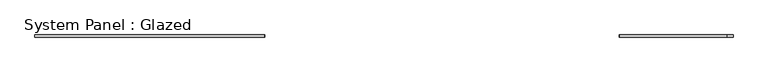
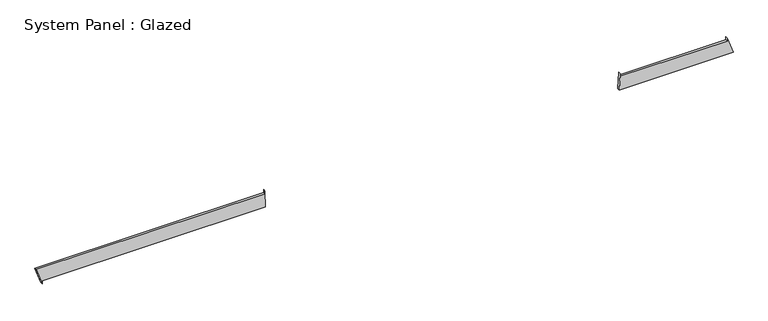
"""IFC4 building model written with IfcOpenShell, lengths in millimetres: plate geometry, System Panel : Glazed."""

import ifcopenshell
import ifcopenshell.guid

model = None  # the IFC model being written
_history = None  # IfcOwnerHistory: only IFC2X3 demands one
_inside = {}  # id of a spatial element -> (the spatial element, [elements in it])
_under = {}  # id of a project, library or spatial element -> (it, [spatial elements below it])
_declared = {}  # id of a project -> (the project, [libraries it declares])
_typed = {}  # id of a type object -> (the type object, [elements of that type])
_made_of = {}  # id of a material, layer set ... -> (it, [elements and type objects made of it])


def new_model(schema):
    """Start an empty IFC model of exactly this schema.

    Asked for "IFC4X3", IfcOpenShell would pick the latest addendum, in which some entities
    have other attributes; the version numbers below select the first issue.
    IFC2X3 requires an IfcOwnerHistory on every rooted entity: one is made here for all.
    """
    global model, _history
    if schema == "IFC4X3":
        model = ifcopenshell.file(schema_version=(4, 3, 0, 0))
    else:
        model = ifcopenshell.file(schema=schema)
    _inside.clear()
    _under.clear()
    _declared.clear()
    _typed.clear()
    _made_of.clear()
    _history = None
    if model.schema == "IFC2X3":
        org = make("IfcOrganization", Name="unknown")
        user = make(
            "IfcPersonAndOrganization",
            ThePerson=make("IfcPerson", FamilyName="unknown"),
            TheOrganization=org,
        )
        app = make(
            "IfcApplication",
            ApplicationDeveloper=org,
            Version="unknown",
            ApplicationFullName="unknown",
            ApplicationIdentifier="unknown",
        )
        _history = make(
            "IfcOwnerHistory",
            OwningUser=user,
            OwningApplication=app,
            ChangeAction="ADDED",
            CreationDate=0,
        )
    return model


def make(cls, **values):
    """One entity of the class cls with the attributes given. An attribute that is None is left unset."""
    return model.create_entity(
        cls, **{name: value for name, value in values.items() if value is not None}
    )


def rooted(cls, **values):
    """An entity with a GlobalId (a new one), such as an element, a storey or a relation."""
    return make(cls, GlobalId=ifcopenshell.guid.new(), OwnerHistory=_history, **values)


def si_unit(unit_type, name, prefix=None):
    """IfcSIUnit, for example si_unit("LENGTHUNIT", "METRE", prefix="MILLI")."""
    return make("IfcSIUnit", UnitType=unit_type, Prefix=prefix, Name=name)


def assignment(units):
    """IfcUnitAssignment: the units of a project."""
    return None if units is None else make("IfcUnitAssignment", Units=units)


def point(xyz):
    """IfcCartesianPoint."""
    return None if xyz is None else make("IfcCartesianPoint", Coordinates=xyz)


def direction(xyz):
    """IfcDirection."""
    return None if xyz is None else make("IfcDirection", DirectionRatios=xyz)


def frame(location, z_axis=None, x_axis=None):
    """IfcAxis2Placement3D, a coordinate frame: its origin and axes. An axis left out is left unset."""
    return make(
        "IfcAxis2Placement3D",
        Location=point(location),
        Axis=direction(z_axis),
        RefDirection=direction(x_axis),
    )


def origin():
    """The frame at (0, 0, 0) with its axes left unset."""
    return frame((0.0, 0.0, 0.0))


def place(relative_to, where):
    """IfcLocalPlacement: puts the frame where relative to a parent placement (None: the world)."""
    return make(
        "IfcLocalPlacement", PlacementRelTo=relative_to, RelativePlacement=where
    )


def context(
    kind, dimensions, precision=None, world=None, true_north=None, identifier=None
):
    """IfcGeometricRepresentationContext, for example the 3D "Model" context."""
    return make(
        "IfcGeometricRepresentationContext",
        ContextIdentifier=identifier,
        ContextType=kind,
        CoordinateSpaceDimension=dimensions,
        Precision=precision,
        WorldCoordinateSystem=world,
        TrueNorth=true_north,
    )


def project(units=None, contexts=None):
    """IfcProject with its units and contexts."""
    return rooted(
        "IfcProject",
        Name="project",
        RepresentationContexts=contexts,
        UnitsInContext=assignment(units),
    )


def spatial(cls, under=None, at=None, **own):
    """A site, building, storey or space (cls), placed at a placement, below another one or the project."""
    s = rooted(cls, ObjectPlacement=at, **own)
    if under is not None:
        _under.setdefault(under.id(), (under, []))[1].append(s)
    return s


def polyline(points):
    """IfcPolyline through the points."""
    return make("IfcPolyline", Points=[point(p) for p in points])


def outline(outer, holes=None, kind="AREA"):
    """IfcArbitraryClosedProfileDef: a profile drawn as a closed curve; with holes, ...WithVoids."""
    if holes is None:
        return make("IfcArbitraryClosedProfileDef", ProfileType=kind, OuterCurve=outer)
    return make(
        "IfcArbitraryProfileDefWithVoids",
        ProfileType=kind,
        OuterCurve=outer,
        InnerCurves=holes,
    )


def extrude(swept, where, along, depth):
    """IfcExtrudedAreaSolid: the profile swept, set in the frame where, extruded along a direction by depth."""
    return make(
        "IfcExtrudedAreaSolid",
        SweptArea=swept,
        Position=where,
        ExtrudedDirection=direction(along),
        Depth=depth,
    )


def shape(context_of_items, identifier, shape_type, items):
    """IfcShapeRepresentation: the items that make up one representation, for example the "Body"."""
    return make(
        "IfcShapeRepresentation",
        ContextOfItems=context_of_items,
        RepresentationIdentifier=identifier,
        RepresentationType=shape_type,
        Items=items,
    )


def source(mapping_origin, context_of_items, identifier, shape_type, items):
    """IfcRepresentationMap: a shape defined once, which mapped items show again and again."""
    return make(
        "IfcRepresentationMap",
        MappingOrigin=mapping_origin,
        MappedRepresentation=shape(context_of_items, identifier, shape_type, items),
    )


def transform(
    local_origin,
    x_axis=None,
    y_axis=None,
    z_axis=None,
    scale=None,
    scale2=None,
    scale3=None,
    uniform=True,
):
    """IfcCartesianTransformationOperator3D, or its non-uniform kind. x_axis, y_axis, z_axis: its Axis1, 2, 3."""
    if uniform:
        return make(
            "IfcCartesianTransformationOperator3D",
            Axis1=direction(x_axis),
            Axis2=direction(y_axis),
            LocalOrigin=point(local_origin),
            Scale=scale,
            Axis3=direction(z_axis),
        )
    return make(
        "IfcCartesianTransformationOperator3DnonUniform",
        Axis1=direction(x_axis),
        Axis2=direction(y_axis),
        LocalOrigin=point(local_origin),
        Scale=scale,
        Axis3=direction(z_axis),
        Scale2=scale2,
        Scale3=scale3,
    )


def mapped(mapping_source, mapping_target):
    """IfcMappedItem: shows the shape of a source again, moved by a transform."""
    return make(
        "IfcMappedItem", MappingSource=mapping_source, MappingTarget=mapping_target
    )


def made_of(thing, what):
    """Note that an element or type object is made of a material, layer set ...; save() writes the relation."""
    if what is not None:
        _made_of.setdefault(what.id(), (what, []))[1].append(thing)
    return thing


def element(
    cls,
    number,
    at=None,
    inside=None,
    cuts=None,
    type_object=None,
    material=None,
    context=None,
    identifier="Body",
    shape_type=None,
    held_by="IfcProductDefinitionShape",
    body=None,
    shapes=None,
    **own,
):
    """One element of the class cls, such as IfcWall. Its Tag is "e" and its number.

    at: its placement. inside: the storey or other place that contains it. cuts: it is an
    opening in that element (IfcRelVoidsElement). A single representation is given by context,
    identifier, shape_type and body (its items); several are given by shapes. held_by: the class
    of the entity that holds the representations. save() writes the other relations.
    """
    e = rooted(cls, Tag="e%d" % number, ObjectPlacement=at, **own)
    if body is not None:
        shapes = [shape(context, identifier, shape_type, body)]
    if shapes is not None:
        e.Representation = make(held_by, Representations=shapes)
    if inside is not None:
        _inside.setdefault(inside.id(), (inside, []))[1].append(e)
    if cuts is not None:
        rooted(
            "IfcRelVoidsElement", RelatingBuildingElement=cuts, RelatedOpeningElement=e
        )
    if type_object is not None:
        _typed.setdefault(type_object.id(), (type_object, []))[1].append(e)
    return made_of(e, material)


def aggregate(whole, parts):
    """IfcRelAggregates: a whole, such as a stair, and the parts it consists of."""
    return rooted("IfcRelAggregates", RelatingObject=whole, RelatedObjects=parts)


def save(model, path):
    """Write the relations noted so far, then the file.

    IfcRelAggregates (storeys below a building ...), IfcRelContainedInSpatialStructure (elements
    in a storey), IfcRelDefinesByType, IfcRelAssociatesMaterial and IfcRelDeclares: one each for
    every whole, place, type object, material and project.
    """
    for whole, parts in _under.values():
        aggregate(whole, parts)
    for where, things in _inside.values():
        rooted(
            "IfcRelContainedInSpatialStructure",
            RelatedElements=things,
            RelatingStructure=where,
        )
    for kind, things in _typed.values():
        rooted("IfcRelDefinesByType", RelatedObjects=things, RelatingType=kind)
    for what, things in _made_of.values():
        rooted("IfcRelAssociatesMaterial", RelatedObjects=things, RelatingMaterial=what)
    for by, libraries in _declared.values():
        rooted("IfcRelDeclares", RelatingContext=by, RelatedDefinitions=libraries)
    model.write(path)


def system_panel_glazed_a1e72640(model_context):
    return source(origin(), model_context, "Body", "SweptSolid", [
        extrude(outline(polyline([(0.0, -3958.5507161), (35.3553391, -3958.5507161), (35.3553391, -1377.5436269), (234.6939562, -1382.7201119), (199.3386172, -1382.7194789), (199.2912695, -4027.4801939), (0.0, -3958.5507161)])), frame((0.0, -49.5, 0.0), z_axis=(0.0, 1.0, 0.0), x_axis=(0.0, 0.0, 1.0)), (0.0, 0.0, 1.0), 25.0),
        extrude(outline(polyline([(35.3553391, 2711.6809934), (35.3553391, 4027.4801939), (234.7895843, 3958.8960097), (199.4342452, 3958.8966426), (199.4121015, 2721.9901772), (234.7674406, 2721.9895442), (35.3553391, 2711.6809934)])), frame((0.0, -49.5, 0.0), z_axis=(0.0, 1.0, 0.0), x_axis=(0.0, 0.0, 1.0)), (0.0, 0.0, 1.0), 25.0),
    ])


if __name__ == "__main__":
    model = new_model("IFC4")
    model_context = context("Model", 3, world=origin())
    ifc_project = project(units=[si_unit("LENGTHUNIT", "METRE", prefix="MILLI")], contexts=[model_context])
    site = spatial("IfcSite", under=ifc_project)
    building = spatial("IfcBuilding", under=site)
    placement = place(None, origin())
    system_panel_glazed_shape = system_panel_glazed_a1e72640(model_context)
    element("IfcPlate", 1, ObjectType="System Panel : Glazed", at=placement, inside=building, context=model_context, shape_type="MappedRepresentation", body=[
        mapped(system_panel_glazed_shape, transform((0.0, 0.0, 0.0), x_axis=(1.0, 0.0, 0.0), y_axis=(0.0, 1.0, 0.0), z_axis=(0.0, 0.0, 1.0))),
    ])
    save(model, "model.ifc")

# Revit data of these elements
# Element 1 (IfcPlate, "System Panel : Glazed")
#   Materials on its faces: "Glass"
# Materials
#   "Glass": class "Glass", colour RGB 218 227 224, transparency 0.85, Description = "Soda Lime Glass", Cost = 0
